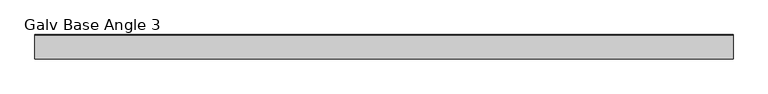
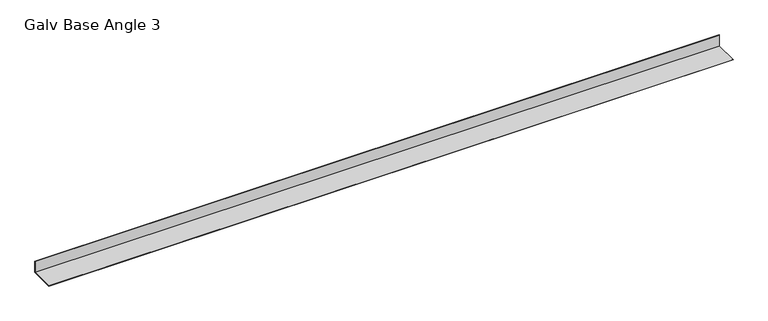
"""IFC4 building model written with IfcOpenShell, lengths in millimetres: proxy geometry, Galv Base Angle 3 : CF Galv L 4x2x16ga."""

from ifc_helpers import new_model, si_unit, frame, origin, place, context, project, spatial, polyline, outline, extrude, source, transform, mapped, element, save


def galv_base_angle_3_bf8ff121(model_context):
    return source(origin(), model_context, "Body", "SweptSolid", [
        extrude(outline(polyline([(-531741.6101341, 0.93726), (-531640.9473941, 0.93726), (-531640.9473941, 50.8), (-531640.0101341, 50.8), (-531640.0101341, 0.0), (-531741.6101341, 0.0), (-531741.6101341, 0.93726)])), frame((587411.9309739, 0.0, 0.0), z_axis=(1.0, 0.0, 0.0), x_axis=(0.0, 1.0, 0.0)), (0.0, 0.0, 1.0), 2906.7125),
    ])


if __name__ == "__main__":
    model = new_model("IFC4")
    model_context = context("Model", 3, world=origin())
    ifc_project = project(units=[si_unit("LENGTHUNIT", "METRE", prefix="MILLI")], contexts=[model_context])
    site = spatial("IfcSite", under=ifc_project)
    building = spatial("IfcBuilding", under=site)
    placement = place(None, origin())
    galv_base_angle_3_shape = galv_base_angle_3_bf8ff121(model_context)
    element("IfcBuildingElementProxy", 1, Name="Galv Base Angle 3 : CF Galv L 4x2x16ga", ObjectType="Galv Base Angle 3 : CF Galv L 4x2x16ga", at=placement, inside=building, context=model_context, shape_type="MappedRepresentation", body=[
        mapped(galv_base_angle_3_shape, transform((0.0, 0.0, 0.0), x_axis=(1.0, 0.0, 0.0), y_axis=(0.0, 1.0, 0.0), z_axis=(0.0, 0.0, 1.0))),
    ])
    save(model, "model.ifc")

# Revit data of these elements
# Element 1 (IfcBuildingElementProxy, "Galv Base Angle 3 : CF Galv L 4x2x16ga")
#   Materials on its faces: "4\"X2\" L - COLD-FORMED GALV."
# Materials
#   "4\"X2\" L - COLD-FORMED GALV.": class "Generic", colour RGB 143 142 141, transparency 0, Cost = 0
